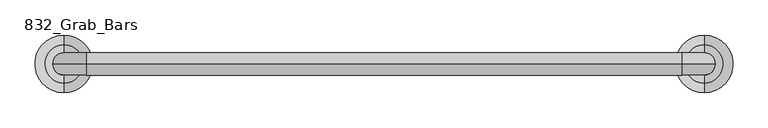
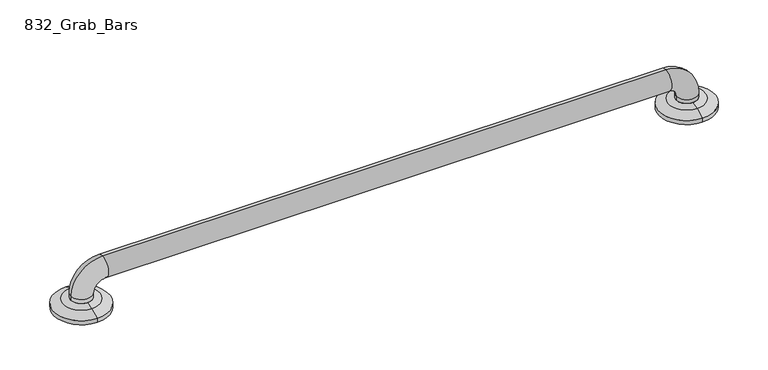
"""IFC4 building model written with IfcOpenShell, lengths in millimetres: proxy geometry, 832_Grab_Bars : 8320-001360."""

from ifc_helpers import new_model, si_unit, point, frame, origin, place, context, project, spatial, polyline, circle_curve, ellipse_curve, trimmed, source, transform, mapped, element, save
from ifc_brep_helpers import plane_surface, cylinder_surface, revolved_surface, advanced_brep


def proxy_832_grab_bars_51fee9e1(model_context):
    return source(origin(), model_context, "Body", "AdvancedBrep", [
        advanced_brep(
        [(-363.5375, -564.1630987, 13.1934507), (-363.5375, -508.9869013, 13.1934507), (-363.5375, -495.3, 6.35), (-363.5375, -577.85, 6.35), (-363.5375, -552.8038734, 15.875), (-363.5375, -520.3461266, 15.875), (-363.5375, -552.45, 15.875), (-379.4125, -536.575, 15.875), (-363.5375, -520.7, 15.875), (-347.6625, -536.575, 15.875), (-363.5375, -577.85, 0.0), (-363.5375, -495.3, 0.0), (-363.5375, -520.7, 0.0), (-363.5375, -536.575, 0.0), (-363.5375, -552.45, 0.0), (550.8625, -564.2276895, 13.1934507), (550.8625, -509.0514921, 13.1934507), (550.8625, -495.3645908, 6.35), (550.8625, -577.9145908, 6.35), (550.8625, -552.8684641, 15.875), (550.8625, -520.4107174, 15.875), (550.8625, -552.45, 15.875), (534.9875, -536.575, 15.875), (550.8625, -520.7, 15.875), (566.7375, -536.575, 15.875), (550.8625, -577.9145908, 0.0), (550.8625, -495.3645908, 0.0), (550.8625, -520.7, 0.0), (550.8625, -536.6395908, 0.0), (550.8625, -552.45, 0.0), (-379.4125, -536.575, 22.225), (-347.6625, -536.575, 22.225), (-331.7875, -536.575, 69.85), (-331.7875, -536.575, 38.1), (519.1125, -536.575, 69.85), (519.1125, -536.575, 38.1), (566.7375, -536.575, 22.225), (534.9875, -536.575, 22.225)],
        [
            (0, 1, circle_curve(frame((-363.5375, -536.575, 13.1934507), z_axis=(0.0, 0.0, -1.0), x_axis=(0.0, 1.0, 0.0)), 27.5880987)),
            (1, 2),
            (2, 3, circle_curve(frame((-363.5375, -536.575, 6.35), z_axis=(0.0, 0.0, 1.0), x_axis=(0.0, 1.0, 0.0)), 41.275)),
            (3, 0),
            (1, 0, circle_curve(frame((-363.5375, -536.575, 13.1934507), z_axis=(0.0, 0.0, -1.0), x_axis=(0.0, 1.0, 0.0)), 27.5880987)),
            (3, 2, circle_curve(frame((-363.5375, -536.575, 6.35), z_axis=(0.0, 0.0, 1.0), x_axis=(0.0, 1.0, 0.0)), 41.275)),
            (0, 4, circle_curve(frame((-363.5375, -552.8038734, -9.525), z_axis=(-1.0, 0.0, 0.0), x_axis=(0.0, 0.0, -1.0)), 25.4)),
            (4, 5, circle_curve(frame((-363.5375, -536.575, 15.875), z_axis=(0.0, 0.0, -1.0), x_axis=(0.0, 1.0, 0.0)), 16.2288734)),
            (5, 1, circle_curve(frame((-363.5375, -520.3461266, -9.525), z_axis=(-1.0, 0.0, 0.0), x_axis=(0.0, 0.0, -1.0)), 25.4)),
            (5, 4, circle_curve(frame((-363.5375, -536.575, 15.875), z_axis=(0.0, 0.0, -1.0), x_axis=(0.0, 1.0, 0.0)), 16.2288734)),
            (4, 6),
            (6, 7, circle_curve(frame((-363.5375, -536.575, 15.875), z_axis=(0.0, 0.0, -1.0), x_axis=(1.0, 0.0, 0.0)), 15.875)),
            (7, 8, circle_curve(frame((-363.5375, -536.575, 15.875), z_axis=(0.0, 0.0, -1.0), x_axis=(1.0, 0.0, 0.0)), 15.875)),
            (8, 5),
            (8, 9, circle_curve(frame((-363.5375, -536.575, 15.875), z_axis=(0.0, 0.0, -1.0), x_axis=(1.0, 0.0, 0.0)), 15.875)),
            (9, 6, circle_curve(frame((-363.5375, -536.575, 15.875), z_axis=(0.0, 0.0, -1.0), x_axis=(1.0, 0.0, 0.0)), 15.875)),
            (10, 11, circle_curve(frame((-363.5375, -536.575, 0.0), z_axis=(0.0, 0.0, -1.0), x_axis=(0.0, 1.0, 0.0)), 41.275)),
            (11, 12),
            (12, 13),
            (13, 14),
            (14, 10),
            (11, 10, circle_curve(frame((-363.5375, -536.575, 0.0), z_axis=(0.0, 0.0, -1.0), x_axis=(0.0, 1.0, 0.0)), 41.275)),
            (2, 11),
            (10, 3),
            (15, 16, circle_curve(frame((550.8625, -536.6395908, 13.1934507), z_axis=(0.0, 0.0, -1.0), x_axis=(0.0, 1.0, 0.0)), 27.5880987)),
            (16, 17),
            (17, 18, circle_curve(frame((550.8625, -536.6395908, 6.35), z_axis=(0.0, 0.0, 1.0), x_axis=(0.0, 1.0, 0.0)), 41.275)),
            (18, 15),
            (16, 15, circle_curve(frame((550.8625, -536.6395908, 13.1934507), z_axis=(0.0, 0.0, -1.0), x_axis=(0.0, 1.0, 0.0)), 27.5880987)),
            (18, 17, circle_curve(frame((550.8625, -536.6395908, 6.35), z_axis=(0.0, 0.0, 1.0), x_axis=(0.0, 1.0, 0.0)), 41.275)),
            (15, 19, circle_curve(frame((550.8625, -552.8684641, -9.525), z_axis=(-1.0, 0.0, 0.0), x_axis=(0.0, 0.0, -1.0)), 25.4)),
            (19, 20, circle_curve(frame((550.8625, -536.6395908, 15.875), z_axis=(0.0, 0.0, -1.0), x_axis=(0.0, 1.0, 0.0)), 16.2288734)),
            (20, 16, circle_curve(frame((550.8625, -520.4107174, -9.525), z_axis=(-1.0, 0.0, 0.0), x_axis=(0.0, 0.0, -1.0)), 25.4)),
            (20, 19, circle_curve(frame((550.8625, -536.6395908, 15.875), z_axis=(0.0, 0.0, -1.0), x_axis=(0.0, 1.0, 0.0)), 16.2288734)),
            (19, 21),
            (21, 22, circle_curve(frame((550.8625, -536.575, 15.875), z_axis=(0.0, 0.0, -1.0), x_axis=(-1.0, 0.0, 0.0)), 15.875)),
            (22, 23, circle_curve(frame((550.8625, -536.575, 15.875), z_axis=(0.0, 0.0, -1.0), x_axis=(-1.0, 0.0, 0.0)), 15.875)),
            (23, 20),
            (23, 24, circle_curve(frame((550.8625, -536.575, 15.875), z_axis=(0.0, 0.0, -1.0), x_axis=(-1.0, 0.0, 0.0)), 15.875)),
            (24, 21, circle_curve(frame((550.8625, -536.575, 15.875), z_axis=(0.0, 0.0, -1.0), x_axis=(-1.0, 0.0, 0.0)), 15.875)),
            (25, 26, circle_curve(frame((550.8625, -536.6395908, 0.0), z_axis=(0.0, 0.0, -1.0), x_axis=(0.0, 1.0, 0.0)), 41.275)),
            (26, 27),
            (27, 28),
            (28, 29),
            (29, 25),
            (26, 25, circle_curve(frame((550.8625, -536.6395908, 0.0), z_axis=(0.0, 0.0, -1.0), x_axis=(0.0, 1.0, 0.0)), 41.275)),
            (17, 26),
            (25, 18),
            (30, 31, circle_curve(frame((-363.5375, -536.575, 22.225), z_axis=(0.0, 0.0, -1.0), x_axis=(1.0, 0.0, 0.0)), 15.875)),
            (31, 9),
            (7, 30),
            (31, 30, circle_curve(frame((-363.5375, -536.575, 22.225), z_axis=(0.0, 0.0, -1.0), x_axis=(1.0, 0.0, 0.0)), 15.875)),
            (30, 32, circle_curve(frame((-331.7875, -536.575, 22.225), z_axis=(0.0, 1.0, 0.0), x_axis=(-1.0, 0.0, 0.0)), 47.625)),
            (32, 33, circle_curve(frame((-331.7875, -536.575, 53.975), z_axis=(-1.0, 0.0, 0.0), x_axis=(0.0, 0.0, -1.0)), 15.875)),
            (33, 31, circle_curve(frame((-331.7875, -536.575, 22.225), z_axis=(0.0, -1.0, 0.0), x_axis=(-1.0, 0.0, 0.0)), 15.875)),
            (33, 32, circle_curve(frame((-331.7875, -536.575, 53.975), z_axis=(-1.0, 0.0, 0.0), x_axis=(0.0, 0.0, -1.0)), 15.875)),
            (32, 34),
            (34, 35, circle_curve(frame((519.1125, -536.575, 53.975), z_axis=(-1.0, 0.0, 0.0), x_axis=(0.0, 0.0, -1.0)), 15.875)),
            (35, 33),
            (35, 34, circle_curve(frame((519.1125, -536.575, 53.975), z_axis=(-1.0, 0.0, 0.0), x_axis=(0.0, 0.0, -1.0)), 15.875)),
            (34, 36, circle_curve(frame((519.1125, -536.575, 22.225), z_axis=(0.0, 1.0, 0.0), x_axis=(0.0, 0.0, 1.0)), 47.625)),
            (36, 37, circle_curve(frame((550.8625, -536.575, 22.225), z_axis=(0.0, 0.0, 1.0), x_axis=(-1.0, 0.0, 0.0)), 15.875)),
            (37, 35, circle_curve(frame((519.1125, -536.575, 22.225), z_axis=(0.0, -1.0, 0.0), x_axis=(0.0, 0.0, 1.0)), 15.875)),
            (37, 36, circle_curve(frame((550.8625, -536.575, 22.225), z_axis=(0.0, 0.0, 1.0), x_axis=(-1.0, 0.0, 0.0)), 15.875)),
            (36, 24),
            (22, 37),
        ],
        [
            revolved_surface(polyline([(-363.5375, -495.3, 6.35), (-363.5375, -508.9869013, 13.1934507)]), (-363.5375, -536.575, 31.75), (0.0, 0.0, 1.0)),
            revolved_surface(trimmed(ellipse_curve(frame((-363.5375, -520.3461266, -9.525), z_axis=(1.0, 0.0, 0.0), x_axis=(0.0, 0.0, -1.0)), 25.4, 25.4), [point((-363.5375, -508.9869013, 13.1934507))], [point((-363.5375, -520.3461266, 15.875))], True, "CARTESIAN"), (-363.5375, -536.575, 31.75), (0.0, 0.0, 1.0)),
            plane_surface(frame((-363.5375, -536.575, 15.875), z_axis=(0.0, 0.0, 1.0), x_axis=(0.0, 1.0, 0.0))),
            plane_surface(frame((-363.5375, -536.575, 0.0), z_axis=(0.0, 0.0, -1.0), x_axis=(0.0, 1.0, 0.0))),
            cylinder_surface(frame((-363.5375, -536.575, 31.75), z_axis=(0.0, 0.0, 1.0), x_axis=(0.0, 1.0, 0.0)), 41.275),
            revolved_surface(polyline([(550.8625, -495.3645908, 6.35), (550.8625, -509.0514921, 13.1934507)]), (550.8625, -536.6395908, 31.75), (0.0, 0.0, 1.0)),
            revolved_surface(trimmed(ellipse_curve(frame((550.8625, -520.4107174, -9.525), z_axis=(1.0, 0.0, 0.0), x_axis=(0.0, 0.0, -1.0)), 25.4, 25.4), [point((550.8625, -509.0514921, 13.1934507))], [point((550.8625, -520.4107174, 15.875))], True, "CARTESIAN"), (550.8625, -536.6395908, 31.75), (0.0, 0.0, 1.0)),
            plane_surface(frame((550.8625, -536.6395908, 15.875), z_axis=(0.0, 0.0, 1.0), x_axis=(0.0, 1.0, 0.0))),
            plane_surface(frame((550.8625, -536.6395908, 0.0), z_axis=(0.0, 0.0, -1.0), x_axis=(0.0, 1.0, 0.0))),
            cylinder_surface(frame((550.8625, -536.6395908, 31.75), z_axis=(0.0, 0.0, 1.0), x_axis=(0.0, 1.0, 0.0)), 41.275),
            cylinder_surface(frame((-363.5375, -536.575, 0.0), z_axis=(0.0, 0.0, -1.0), x_axis=(1.0, 0.0, 0.0)), 15.875),
            revolved_surface(trimmed(ellipse_curve(frame((-363.5375, -536.575, 22.225), z_axis=(0.0, 0.0, -1.0), x_axis=(1.0, 0.0, 0.0)), 15.875, 15.875), [point((-379.4125, -536.575, 22.225))], [point((-347.6625, -536.575, 22.225))], True, "CARTESIAN"), (-331.7875, -536.575, 22.225), (0.0, 1.0, 0.0)),
            revolved_surface(trimmed(ellipse_curve(frame((-363.5375, -536.575, 22.225), z_axis=(0.0, 0.0, -1.0), x_axis=(1.0, 0.0, 0.0)), 15.875, 15.875), [point((-347.6625, -536.575, 22.225))], [point((-379.4125, -536.575, 22.225))], True, "CARTESIAN"), (-331.7875, -536.575, 22.225), (0.0, 1.0, 0.0)),
            cylinder_surface(frame((-331.7875, -536.575, 53.975), z_axis=(-1.0, 0.0, 0.0), x_axis=(0.0, 0.0, -1.0)), 15.875),
            revolved_surface(trimmed(ellipse_curve(frame((519.1125, -536.575, 53.975), z_axis=(-1.0, 0.0, 0.0), x_axis=(0.0, 0.0, -1.0)), 15.875, 15.875), [point((519.1125, -536.575, 69.85))], [point((519.1125, -536.575, 38.1))], True, "CARTESIAN"), (519.1125, -536.575, 22.225), (0.0, 1.0, 0.0)),
            revolved_surface(trimmed(ellipse_curve(frame((519.1125, -536.575, 53.975), z_axis=(-1.0, 0.0, 0.0), x_axis=(0.0, 0.0, -1.0)), 15.875, 15.875), [point((519.1125, -536.575, 38.1))], [point((519.1125, -536.575, 69.85))], True, "CARTESIAN"), (519.1125, -536.575, 22.225), (0.0, 1.0, 0.0)),
            cylinder_surface(frame((550.8625, -536.575, 22.225), z_axis=(0.0, 0.0, 1.0), x_axis=(-1.0, 0.0, 0.0)), 15.875),
        ],
        [
            (0, [[1, 2, 3, 4]]),
            (0, [[-2, 5, -4, 6]]),
            (1, [[-1, 7, 8, 9]]),
            (1, [[-5, -9, 10, -7]]),
            (2, [[-8, 11, 12, 13, 14]]),
            (2, [[-10, -14, 15, 16, -11]]),
            (3, [[17, 18, 19, 20, 21]]),
            (3, [[22, -21, -20, -19, -18]]),
            (4, [[-3, 23, -17, 24]]),
            (4, [[-6, -24, -22, -23]]),
            (5, [[25, 26, 27, 28]]),
            (5, [[-26, 29, -28, 30]]),
            (6, [[-25, 31, 32, 33]]),
            (6, [[-29, -33, 34, -31]]),
            (7, [[-32, 35, 36, 37, 38]]),
            (7, [[-34, -38, 39, 40, -35]]),
            (8, [[41, 42, 43, 44, 45]]),
            (8, [[46, -45, -44, -43, -42]]),
            (9, [[-27, 47, -41, 48]]),
            (9, [[-30, -48, -46, -47]]),
            (10, [[49, 50, -15, -13, 51]]),
            (10, [[52, -51, -12, -16, -50]]),
            (11, [[-49, 53, 54, 55]]),
            (12, [[-52, -55, 56, -53]]),
            (13, [[-54, 57, 58, 59]]),
            (13, [[-56, -59, 60, -57]]),
            (14, [[-58, 61, 62, 63]]),
            (15, [[-60, -63, 64, -61]]),
            (16, [[-62, 65, -39, -37, 66]]),
            (16, [[-64, -66, -36, -40, -65]]),
        ],
    ),
    ])


if __name__ == "__main__":
    model = new_model("IFC4")
    model_context = context("Model", 3, world=origin())
    ifc_project = project(units=[si_unit("LENGTHUNIT", "METRE", prefix="MILLI")], contexts=[model_context])
    site = spatial("IfcSite", under=ifc_project)
    building = spatial("IfcBuilding", under=site)
    placement = place(None, origin())
    proxy_832_grab_bars_shape = proxy_832_grab_bars_51fee9e1(model_context)
    element("IfcBuildingElementProxy", 1, Name="832_Grab_Bars : 8320-001360", ObjectType="832_Grab_Bars : 8320-001360", at=placement, inside=building, context=model_context, shape_type="MappedRepresentation", body=[
        mapped(proxy_832_grab_bars_shape, transform((0.0, 0.0, 0.0), x_axis=(1.0, 0.0, 0.0), y_axis=(0.0, 1.0, 0.0), z_axis=(0.0, 0.0, 1.0))),
    ])
    save(model, "model.ifc")

# Revit data of these elements
# Type "832_Grab_Bars : 8320-001360"
#   Warranty Information = "Complete unit, one (1) year"
#   Version = "1.0"
#   Technical Data = "http://www.bradleycorp.com/products/techdata/8820.pdf"
#   URL = "www.bradleycorp.com"
#   Type Comments = "All grab bar configurations are specified using centerline to centerline dimensions."
#   OmniClass Title = ""
#   Modeling Code = ""
#   Model = "8320-001360"
#   Material Note = "FLANGES - 13GA., ESCUTCHEONS - 22GA., TUBING - 18GA."
#   MasterFormat Section Title = ""
#   Manufacturer = "Bradley Corporation"
#   LEED Credit = ""
#   Instructions [instance default] = "This is a face mounted fixture."
#   Industry Standards = "ANSI Standard A117.1, ADA, ABA, ADAAG, UFAS"
#   Fire Rating = "None"
#   Description = "Grab Bars"
#   Copyright = "This Model Data is Property of Bradley Corporation"
#   Complies to NAFTA = "Yes"
#   Complies To Buy American Act = "Yes"
#   Assembly Code = "C1030200"
#   ADA Compliant = "Yes"
#   Radius = 15.875 mm
#   Percentage of Recycled Content = 64.64
#   Overall Length = 996.95 mm
#   OmniClass Code = 0
#   MasterFormat Section Number = 0
#   Length = 914.4 mm
#   Diameter = 31.75 mm
#   Default Elevation = 838.2 mm
#   Material and Finish = Bradley Corp Stainless Steel - Satin
# Element 1 (IfcBuildingElementProxy, "832_Grab_Bars : 8320-001360")
#   Materials on its faces: "Bradley Corp Stainless Steel - Satin"
# Materials
#   "Bradley Corp Stainless Steel - Satin": class "Metal", colour RGB 189 187 185, transparency 0, Manufacturer = "Bradley Corporation", URL = "www.bradleycorp.com", Description = "Stainless Steel - Satin Finish", Cost = 0
